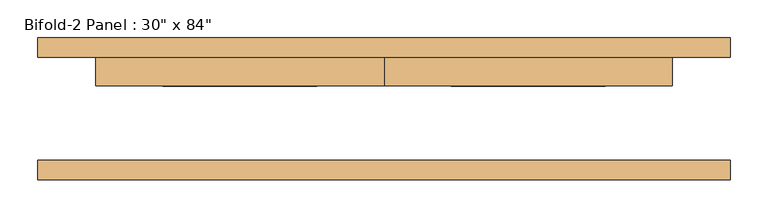
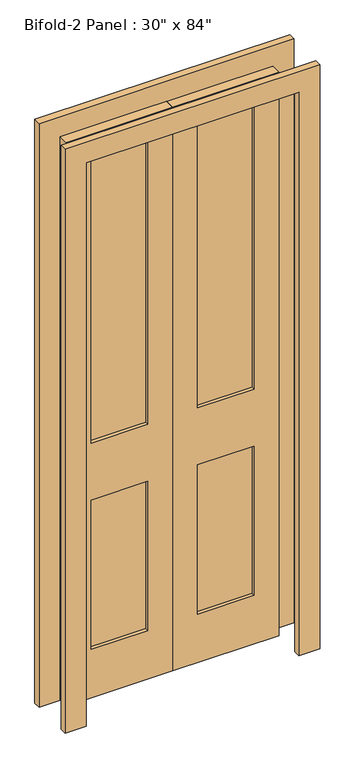
"""IFC4 building model written with IfcOpenShell, lengths in millimetres: door geometry."""

import ifcopenshell
import ifcopenshell.guid

model = None  # the IFC model being written
_history = None  # IfcOwnerHistory: only IFC2X3 demands one
_inside = {}  # id of a spatial element -> (the spatial element, [elements in it])
_under = {}  # id of a project, library or spatial element -> (it, [spatial elements below it])
_declared = {}  # id of a project -> (the project, [libraries it declares])
_typed = {}  # id of a type object -> (the type object, [elements of that type])
_made_of = {}  # id of a material, layer set ... -> (it, [elements and type objects made of it])


def new_model(schema):
    """Start an empty IFC model of exactly this schema.

    Asked for "IFC4X3", IfcOpenShell would pick the latest addendum, in which some entities
    have other attributes; the version numbers below select the first issue.
    IFC2X3 requires an IfcOwnerHistory on every rooted entity: one is made here for all.
    """
    global model, _history
    if schema == "IFC4X3":
        model = ifcopenshell.file(schema_version=(4, 3, 0, 0))
    else:
        model = ifcopenshell.file(schema=schema)
    _inside.clear()
    _under.clear()
    _declared.clear()
    _typed.clear()
    _made_of.clear()
    _history = None
    if model.schema == "IFC2X3":
        org = make("IfcOrganization", Name="unknown")
        user = make(
            "IfcPersonAndOrganization",
            ThePerson=make("IfcPerson", FamilyName="unknown"),
            TheOrganization=org,
        )
        app = make(
            "IfcApplication",
            ApplicationDeveloper=org,
            Version="unknown",
            ApplicationFullName="unknown",
            ApplicationIdentifier="unknown",
        )
        _history = make(
            "IfcOwnerHistory",
            OwningUser=user,
            OwningApplication=app,
            ChangeAction="ADDED",
            CreationDate=0,
        )
    return model


def make(cls, **values):
    """One entity of the class cls with the attributes given. An attribute that is None is left unset."""
    return model.create_entity(
        cls, **{name: value for name, value in values.items() if value is not None}
    )


def rooted(cls, **values):
    """An entity with a GlobalId (a new one), such as an element, a storey or a relation."""
    return make(cls, GlobalId=ifcopenshell.guid.new(), OwnerHistory=_history, **values)


def si_unit(unit_type, name, prefix=None):
    """IfcSIUnit, for example si_unit("LENGTHUNIT", "METRE", prefix="MILLI")."""
    return make("IfcSIUnit", UnitType=unit_type, Prefix=prefix, Name=name)


def assignment(units):
    """IfcUnitAssignment: the units of a project."""
    return None if units is None else make("IfcUnitAssignment", Units=units)


def point(xyz):
    """IfcCartesianPoint."""
    return None if xyz is None else make("IfcCartesianPoint", Coordinates=xyz)


def direction(xyz):
    """IfcDirection."""
    return None if xyz is None else make("IfcDirection", DirectionRatios=xyz)


def frame(location, z_axis=None, x_axis=None):
    """IfcAxis2Placement3D, a coordinate frame: its origin and axes. An axis left out is left unset."""
    return make(
        "IfcAxis2Placement3D",
        Location=point(location),
        Axis=direction(z_axis),
        RefDirection=direction(x_axis),
    )


def origin():
    """The frame at (0, 0, 0) with its axes left unset."""
    return frame((0.0, 0.0, 0.0))


def place(relative_to, where):
    """IfcLocalPlacement: puts the frame where relative to a parent placement (None: the world)."""
    return make(
        "IfcLocalPlacement", PlacementRelTo=relative_to, RelativePlacement=where
    )


def context(
    kind, dimensions, precision=None, world=None, true_north=None, identifier=None
):
    """IfcGeometricRepresentationContext, for example the 3D "Model" context."""
    return make(
        "IfcGeometricRepresentationContext",
        ContextIdentifier=identifier,
        ContextType=kind,
        CoordinateSpaceDimension=dimensions,
        Precision=precision,
        WorldCoordinateSystem=world,
        TrueNorth=true_north,
    )


def project(units=None, contexts=None):
    """IfcProject with its units and contexts."""
    return rooted(
        "IfcProject",
        Name="project",
        RepresentationContexts=contexts,
        UnitsInContext=assignment(units),
    )


def spatial(cls, under=None, at=None, **own):
    """A site, building, storey or space (cls), placed at a placement, below another one or the project."""
    s = rooted(cls, ObjectPlacement=at, **own)
    if under is not None:
        _under.setdefault(under.id(), (under, []))[1].append(s)
    return s


def polyline(points):
    """IfcPolyline through the points."""
    return make("IfcPolyline", Points=[point(p) for p in points])


def outline(outer, holes=None, kind="AREA"):
    """IfcArbitraryClosedProfileDef: a profile drawn as a closed curve; with holes, ...WithVoids."""
    if holes is None:
        return make("IfcArbitraryClosedProfileDef", ProfileType=kind, OuterCurve=outer)
    return make(
        "IfcArbitraryProfileDefWithVoids",
        ProfileType=kind,
        OuterCurve=outer,
        InnerCurves=holes,
    )


def extrude(swept, where, along, depth):
    """IfcExtrudedAreaSolid: the profile swept, set in the frame where, extruded along a direction by depth."""
    return make(
        "IfcExtrudedAreaSolid",
        SweptArea=swept,
        Position=where,
        ExtrudedDirection=direction(along),
        Depth=depth,
    )


def shape(context_of_items, identifier, shape_type, items):
    """IfcShapeRepresentation: the items that make up one representation, for example the "Body"."""
    return make(
        "IfcShapeRepresentation",
        ContextOfItems=context_of_items,
        RepresentationIdentifier=identifier,
        RepresentationType=shape_type,
        Items=items,
    )


def source(mapping_origin, context_of_items, identifier, shape_type, items):
    """IfcRepresentationMap: a shape defined once, which mapped items show again and again."""
    return make(
        "IfcRepresentationMap",
        MappingOrigin=mapping_origin,
        MappedRepresentation=shape(context_of_items, identifier, shape_type, items),
    )


def transform(
    local_origin,
    x_axis=None,
    y_axis=None,
    z_axis=None,
    scale=None,
    scale2=None,
    scale3=None,
    uniform=True,
):
    """IfcCartesianTransformationOperator3D, or its non-uniform kind. x_axis, y_axis, z_axis: its Axis1, 2, 3."""
    if uniform:
        return make(
            "IfcCartesianTransformationOperator3D",
            Axis1=direction(x_axis),
            Axis2=direction(y_axis),
            LocalOrigin=point(local_origin),
            Scale=scale,
            Axis3=direction(z_axis),
        )
    return make(
        "IfcCartesianTransformationOperator3DnonUniform",
        Axis1=direction(x_axis),
        Axis2=direction(y_axis),
        LocalOrigin=point(local_origin),
        Scale=scale,
        Axis3=direction(z_axis),
        Scale2=scale2,
        Scale3=scale3,
    )


def mapped(mapping_source, mapping_target):
    """IfcMappedItem: shows the shape of a source again, moved by a transform."""
    return make(
        "IfcMappedItem", MappingSource=mapping_source, MappingTarget=mapping_target
    )


def made_of(thing, what):
    """Note that an element or type object is made of a material, layer set ...; save() writes the relation."""
    if what is not None:
        _made_of.setdefault(what.id(), (what, []))[1].append(thing)
    return thing


def element(
    cls,
    number,
    at=None,
    inside=None,
    cuts=None,
    type_object=None,
    material=None,
    context=None,
    identifier="Body",
    shape_type=None,
    held_by="IfcProductDefinitionShape",
    body=None,
    shapes=None,
    **own,
):
    """One element of the class cls, such as IfcWall. Its Tag is "e" and its number.

    at: its placement. inside: the storey or other place that contains it. cuts: it is an
    opening in that element (IfcRelVoidsElement). A single representation is given by context,
    identifier, shape_type and body (its items); several are given by shapes. held_by: the class
    of the entity that holds the representations. save() writes the other relations.
    """
    e = rooted(cls, Tag="e%d" % number, ObjectPlacement=at, **own)
    if body is not None:
        shapes = [shape(context, identifier, shape_type, body)]
    if shapes is not None:
        e.Representation = make(held_by, Representations=shapes)
    if inside is not None:
        _inside.setdefault(inside.id(), (inside, []))[1].append(e)
    if cuts is not None:
        rooted(
            "IfcRelVoidsElement", RelatingBuildingElement=cuts, RelatedOpeningElement=e
        )
    if type_object is not None:
        _typed.setdefault(type_object.id(), (type_object, []))[1].append(e)
    return made_of(e, material)


def aggregate(whole, parts):
    """IfcRelAggregates: a whole, such as a stair, and the parts it consists of."""
    return rooted("IfcRelAggregates", RelatingObject=whole, RelatedObjects=parts)


def save(model, path):
    """Write the relations noted so far, then the file.

    IfcRelAggregates (storeys below a building ...), IfcRelContainedInSpatialStructure (elements
    in a storey), IfcRelDefinesByType, IfcRelAssociatesMaterial and IfcRelDeclares: one each for
    every whole, place, type object, material and project.
    """
    for whole, parts in _under.values():
        aggregate(whole, parts)
    for where, things in _inside.values():
        rooted(
            "IfcRelContainedInSpatialStructure",
            RelatedElements=things,
            RelatingStructure=where,
        )
    for kind, things in _typed.values():
        rooted("IfcRelDefinesByType", RelatedObjects=things, RelatingType=kind)
    for what, things in _made_of.values():
        rooted("IfcRelAssociatesMaterial", RelatedObjects=things, RelatingMaterial=what)
    for by, libraries in _declared.values():
        rooted("IfcRelDeclares", RelatingContext=by, RelatedDefinitions=libraries)
    model.write(path)


def door_bb229190(model_context):
    return source(origin(), model_context, "Body", "SweptSolid", [
        extrude(outline(polyline([(2133.6, 0.0), (2133.6, -381.0), (0.0, -381.0), (0.0, 0.0), (2133.6, 0.0)]), holes=[polyline([(2044.7, -88.9), (965.11872, -88.9), (965.11872, -292.1), (2044.7, -292.1), (2044.7, -88.9)]), polyline([(749.3, -88.9), (184.15, -88.9), (184.15, -292.1), (749.3, -292.1), (749.3, -88.9)])]), frame((0.0, 30.1625, 0.0), z_axis=(0.0, 1.0, 0.0), x_axis=(0.0, 0.0, 1.0)), (0.0, 0.0, 1.0), 38.1),
        extrude(outline(polyline([(-88.9, 42.8625), (-292.1, 42.8625), (-292.1, 55.5625), (-88.9, 55.5625), (-88.9, 42.8625)])), frame((0.0, 0.0, 965.11872), z_axis=(0.0, 0.0, 1.0), x_axis=(1.0, 0.0, 0.0)), (0.0, 0.0, 1.0), 1079.58128),
        extrude(outline(polyline([(-88.9, 42.8625), (-292.1, 42.8625), (-292.1, 55.5625), (-88.9, 55.5625), (-88.9, 42.8625)])), frame((0.0, 0.0, 184.15), z_axis=(0.0, 0.0, 1.0), x_axis=(1.0, 0.0, 0.0)), (0.0, 0.0, 1.0), 565.15),
        extrude(outline(polyline([(292.1, 42.8625), (88.9, 42.8625), (88.9, 55.5625), (292.1, 55.5625), (292.1, 42.8625)])), frame((0.0, 0.0, 965.11872), z_axis=(0.0, 0.0, 1.0), x_axis=(1.0, 0.0, 0.0)), (0.0, 0.0, 1.0), 1079.58128),
        extrude(outline(polyline([(292.1, 42.8625), (88.9, 42.8625), (88.9, 55.5625), (292.1, 55.5625), (292.1, 42.8625)])), frame((0.0, 0.0, 184.15), z_axis=(0.0, 0.0, 1.0), x_axis=(1.0, 0.0, 0.0)), (0.0, 0.0, 1.0), 565.15),
        extrude(outline(polyline([(2209.8, -457.2), (0.0, -457.2), (0.0, -381.0), (2133.6, -381.0), (2133.6, 381.0), (0.0, 381.0), (0.0, 457.2), (2209.8, 457.2), (2209.8, -457.2)])), frame((0.0, 68.2625, 0.0), z_axis=(0.0, 1.0, 0.0), x_axis=(0.0, 0.0, 1.0)), (0.0, 0.0, 1.0), 25.4),
        extrude(outline(polyline([(2209.8, 457.2), (2209.8, -457.2), (0.0, -457.2), (0.0, -381.0), (2133.6, -381.0), (2133.6, 381.0), (0.0, 381.0), (0.0, 457.2), (2209.8, 457.2)])), frame((0.0, -93.6625, 0.0), z_axis=(0.0, 1.0, 0.0), x_axis=(0.0, 0.0, 1.0)), (0.0, 0.0, 1.0), 25.4),
        extrude(outline(polyline([(2133.6, 381.0), (2133.6, 0.0), (0.0, 0.0), (0.0, 381.0), (2133.6, 381.0)]), holes=[polyline([(2044.7, 88.9), (2044.7, 292.1), (965.11872, 292.1), (965.11872, 88.9), (2044.7, 88.9)]), polyline([(749.3, 88.9), (749.3, 292.1), (184.15, 292.1), (184.15, 88.9), (749.3, 88.9)])]), frame((0.0, 30.1625, 0.0), z_axis=(0.0, 1.0, 0.0), x_axis=(0.0, 0.0, 1.0)), (0.0, 0.0, 1.0), 38.1),
    ])


if __name__ == "__main__":
    model = new_model("IFC4")
    model_context = context("Model", 3, world=origin())
    ifc_project = project(units=[si_unit("LENGTHUNIT", "METRE", prefix="MILLI")], contexts=[model_context])
    site = spatial("IfcSite", under=ifc_project)
    building = spatial("IfcBuilding", under=site)
    placement = place(None, origin())
    door_shape = door_bb229190(model_context)
    element("IfcDoor", 1, ObjectType="Bifold-2 Panel : 30\" x 84\"", at=placement, inside=building, context=model_context, shape_type="MappedRepresentation", body=[
        mapped(door_shape, transform((0.0, 0.0, 0.0), x_axis=(1.0, 0.0, 0.0), y_axis=(0.0, 1.0, 0.0), z_axis=(0.0, 0.0, 1.0))),
    ])
    save(model, "model.ifc")

# Revit data of these elements
# Type "Bifold-2 Panel : 30\" x 84\""
#   Type Mark = "35"
#   Assembly Code = "C1020"
#   Thickness = 0' - 1 1/2"
#   Height = 7' - 0"
#   Trim Projection Ext = 0' - 1"
#   Trim Projection Int = 0' - 1"
#   Trim Width = 0' - 3"
#   Width = 2' - 6"
#   Door Material = Door - Panel
#   Frame Material = Door - Frame
#   Function = (empty or 0)
#   Wall Closure = (empty or 0)
# Element 1 (IfcDoor, "Bifold-2 Panel : 30\" x 84\"")
#   Materials on its faces: "Door - Panel", "Door - Frame"
# Materials
#   "Door - Panel": class "Wood", colour RGB 210 159 95, transparency 0, Cost = 0
#   "Door - Frame": class "Miscellaneous", colour RGB 118 70 51, transparency 0, Cost = 0
